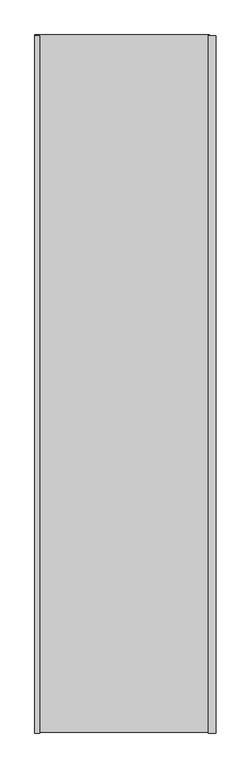
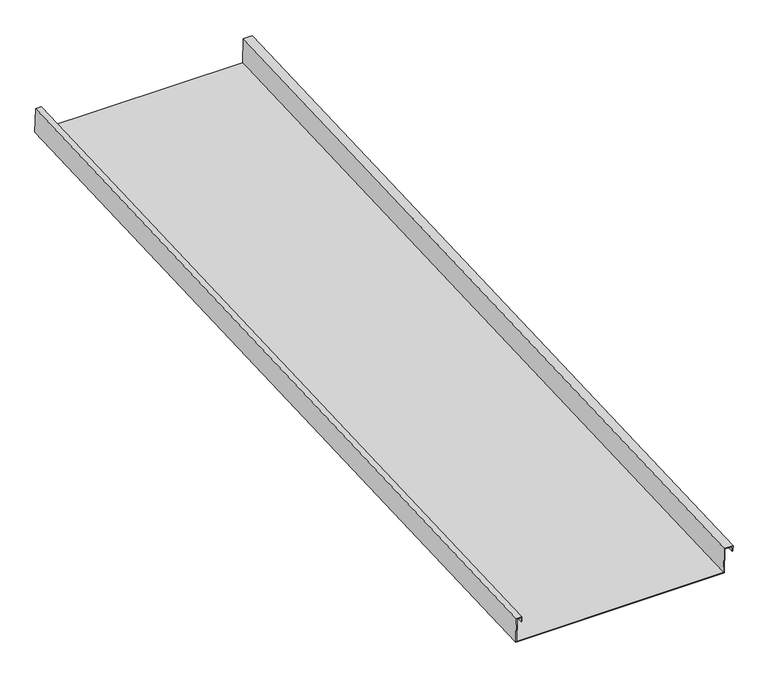
"""IFC4 building model written with IfcOpenShell, lengths in millimetres: proxy geometry, Generic Models 2:Generic Models 2:310765:Generic Models 2:310765 : Generic Models 2:Generic Models 2:310765:62 : Generic Models 2:Generic Models 2:310765:Generic Models 2:310765 : Generic Models 2:Generic Models 2:310765:300385."""

import ifcopenshell
import ifcopenshell.guid

model = None  # the IFC model being written
_history = None  # IfcOwnerHistory: only IFC2X3 demands one
_inside = {}  # id of a spatial element -> (the spatial element, [elements in it])
_under = {}  # id of a project, library or spatial element -> (it, [spatial elements below it])
_declared = {}  # id of a project -> (the project, [libraries it declares])
_typed = {}  # id of a type object -> (the type object, [elements of that type])
_made_of = {}  # id of a material, layer set ... -> (it, [elements and type objects made of it])


def new_model(schema):
    """Start an empty IFC model of exactly this schema.

    Asked for "IFC4X3", IfcOpenShell would pick the latest addendum, in which some entities
    have other attributes; the version numbers below select the first issue.
    IFC2X3 requires an IfcOwnerHistory on every rooted entity: one is made here for all.
    """
    global model, _history
    if schema == "IFC4X3":
        model = ifcopenshell.file(schema_version=(4, 3, 0, 0))
    else:
        model = ifcopenshell.file(schema=schema)
    _inside.clear()
    _under.clear()
    _declared.clear()
    _typed.clear()
    _made_of.clear()
    _history = None
    if model.schema == "IFC2X3":
        org = make("IfcOrganization", Name="unknown")
        user = make(
            "IfcPersonAndOrganization",
            ThePerson=make("IfcPerson", FamilyName="unknown"),
            TheOrganization=org,
        )
        app = make(
            "IfcApplication",
            ApplicationDeveloper=org,
            Version="unknown",
            ApplicationFullName="unknown",
            ApplicationIdentifier="unknown",
        )
        _history = make(
            "IfcOwnerHistory",
            OwningUser=user,
            OwningApplication=app,
            ChangeAction="ADDED",
            CreationDate=0,
        )
    return model


def make(cls, **values):
    """One entity of the class cls with the attributes given. An attribute that is None is left unset."""
    return model.create_entity(
        cls, **{name: value for name, value in values.items() if value is not None}
    )


def rooted(cls, **values):
    """An entity with a GlobalId (a new one), such as an element, a storey or a relation."""
    return make(cls, GlobalId=ifcopenshell.guid.new(), OwnerHistory=_history, **values)


def si_unit(unit_type, name, prefix=None):
    """IfcSIUnit, for example si_unit("LENGTHUNIT", "METRE", prefix="MILLI")."""
    return make("IfcSIUnit", UnitType=unit_type, Prefix=prefix, Name=name)


def assignment(units):
    """IfcUnitAssignment: the units of a project."""
    return None if units is None else make("IfcUnitAssignment", Units=units)


def point(xyz):
    """IfcCartesianPoint."""
    return None if xyz is None else make("IfcCartesianPoint", Coordinates=xyz)


def direction(xyz):
    """IfcDirection."""
    return None if xyz is None else make("IfcDirection", DirectionRatios=xyz)


def frame(location, z_axis=None, x_axis=None):
    """IfcAxis2Placement3D, a coordinate frame: its origin and axes. An axis left out is left unset."""
    return make(
        "IfcAxis2Placement3D",
        Location=point(location),
        Axis=direction(z_axis),
        RefDirection=direction(x_axis),
    )


def origin():
    """The frame at (0, 0, 0) with its axes left unset."""
    return frame((0.0, 0.0, 0.0))


def place(relative_to, where):
    """IfcLocalPlacement: puts the frame where relative to a parent placement (None: the world)."""
    return make(
        "IfcLocalPlacement", PlacementRelTo=relative_to, RelativePlacement=where
    )


def context(
    kind, dimensions, precision=None, world=None, true_north=None, identifier=None
):
    """IfcGeometricRepresentationContext, for example the 3D "Model" context."""
    return make(
        "IfcGeometricRepresentationContext",
        ContextIdentifier=identifier,
        ContextType=kind,
        CoordinateSpaceDimension=dimensions,
        Precision=precision,
        WorldCoordinateSystem=world,
        TrueNorth=true_north,
    )


def project(units=None, contexts=None):
    """IfcProject with its units and contexts."""
    return rooted(
        "IfcProject",
        Name="project",
        RepresentationContexts=contexts,
        UnitsInContext=assignment(units),
    )


def spatial(cls, under=None, at=None, **own):
    """A site, building, storey or space (cls), placed at a placement, below another one or the project."""
    s = rooted(cls, ObjectPlacement=at, **own)
    if under is not None:
        _under.setdefault(under.id(), (under, []))[1].append(s)
    return s


def polyline(points):
    """IfcPolyline through the points."""
    return make("IfcPolyline", Points=[point(p) for p in points])


def outline(outer, holes=None, kind="AREA"):
    """IfcArbitraryClosedProfileDef: a profile drawn as a closed curve; with holes, ...WithVoids."""
    if holes is None:
        return make("IfcArbitraryClosedProfileDef", ProfileType=kind, OuterCurve=outer)
    return make(
        "IfcArbitraryProfileDefWithVoids",
        ProfileType=kind,
        OuterCurve=outer,
        InnerCurves=holes,
    )


def extrude(swept, where, along, depth):
    """IfcExtrudedAreaSolid: the profile swept, set in the frame where, extruded along a direction by depth."""
    return make(
        "IfcExtrudedAreaSolid",
        SweptArea=swept,
        Position=where,
        ExtrudedDirection=direction(along),
        Depth=depth,
    )


def shape(context_of_items, identifier, shape_type, items):
    """IfcShapeRepresentation: the items that make up one representation, for example the "Body"."""
    return make(
        "IfcShapeRepresentation",
        ContextOfItems=context_of_items,
        RepresentationIdentifier=identifier,
        RepresentationType=shape_type,
        Items=items,
    )


def source(mapping_origin, context_of_items, identifier, shape_type, items):
    """IfcRepresentationMap: a shape defined once, which mapped items show again and again."""
    return make(
        "IfcRepresentationMap",
        MappingOrigin=mapping_origin,
        MappedRepresentation=shape(context_of_items, identifier, shape_type, items),
    )


def transform(
    local_origin,
    x_axis=None,
    y_axis=None,
    z_axis=None,
    scale=None,
    scale2=None,
    scale3=None,
    uniform=True,
):
    """IfcCartesianTransformationOperator3D, or its non-uniform kind. x_axis, y_axis, z_axis: its Axis1, 2, 3."""
    if uniform:
        return make(
            "IfcCartesianTransformationOperator3D",
            Axis1=direction(x_axis),
            Axis2=direction(y_axis),
            LocalOrigin=point(local_origin),
            Scale=scale,
            Axis3=direction(z_axis),
        )
    return make(
        "IfcCartesianTransformationOperator3DnonUniform",
        Axis1=direction(x_axis),
        Axis2=direction(y_axis),
        LocalOrigin=point(local_origin),
        Scale=scale,
        Axis3=direction(z_axis),
        Scale2=scale2,
        Scale3=scale3,
    )


def mapped(mapping_source, mapping_target):
    """IfcMappedItem: shows the shape of a source again, moved by a transform."""
    return make(
        "IfcMappedItem", MappingSource=mapping_source, MappingTarget=mapping_target
    )


def made_of(thing, what):
    """Note that an element or type object is made of a material, layer set ...; save() writes the relation."""
    if what is not None:
        _made_of.setdefault(what.id(), (what, []))[1].append(thing)
    return thing


def element(
    cls,
    number,
    at=None,
    inside=None,
    cuts=None,
    type_object=None,
    material=None,
    context=None,
    identifier="Body",
    shape_type=None,
    held_by="IfcProductDefinitionShape",
    body=None,
    shapes=None,
    **own,
):
    """One element of the class cls, such as IfcWall. Its Tag is "e" and its number.

    at: its placement. inside: the storey or other place that contains it. cuts: it is an
    opening in that element (IfcRelVoidsElement). A single representation is given by context,
    identifier, shape_type and body (its items); several are given by shapes. held_by: the class
    of the entity that holds the representations. save() writes the other relations.
    """
    e = rooted(cls, Tag="e%d" % number, ObjectPlacement=at, **own)
    if body is not None:
        shapes = [shape(context, identifier, shape_type, body)]
    if shapes is not None:
        e.Representation = make(held_by, Representations=shapes)
    if inside is not None:
        _inside.setdefault(inside.id(), (inside, []))[1].append(e)
    if cuts is not None:
        rooted(
            "IfcRelVoidsElement", RelatingBuildingElement=cuts, RelatedOpeningElement=e
        )
    if type_object is not None:
        _typed.setdefault(type_object.id(), (type_object, []))[1].append(e)
    return made_of(e, material)


def aggregate(whole, parts):
    """IfcRelAggregates: a whole, such as a stair, and the parts it consists of."""
    return rooted("IfcRelAggregates", RelatingObject=whole, RelatedObjects=parts)


def save(model, path):
    """Write the relations noted so far, then the file.

    IfcRelAggregates (storeys below a building ...), IfcRelContainedInSpatialStructure (elements
    in a storey), IfcRelDefinesByType, IfcRelAssociatesMaterial and IfcRelDeclares: one each for
    every whole, place, type object, material and project.
    """
    for whole, parts in _under.values():
        aggregate(whole, parts)
    for where, things in _inside.values():
        rooted(
            "IfcRelContainedInSpatialStructure",
            RelatedElements=things,
            RelatingStructure=where,
        )
    for kind, things in _typed.values():
        rooted("IfcRelDefinesByType", RelatedObjects=things, RelatingType=kind)
    for what, things in _made_of.values():
        rooted("IfcRelAssociatesMaterial", RelatedObjects=things, RelatingMaterial=what)
    for by, libraries in _declared.values():
        rooted("IfcRelDeclares", RelatingContext=by, RelatedDefinitions=libraries)
    model.write(path)


def generic_models_d106d9bd(model_context):
    return source(origin(), model_context, "Body", "SweptSolid", [
        extrude(outline(polyline([(50.8, 0.0), (50.8, 14.2875), (41.275, 14.2875), (41.275, 15.875), (52.3875, 15.875), (52.3875, -1.5875), (1.5874999, -1.5875), (1.5874999, -404.8125), (47.625, -404.8125), (47.625, -396.875), (39.6875, -396.875), (39.6875, -395.2875), (49.2125, -395.2875), (49.2125, -406.4), (0.0, -406.4), (0.0, 0.0), (50.8, 0.0)])), frame((579172.0218144, -580678.4204475, 3889.8483266), z_axis=(0.0, 0.9991330730923567, 0.04163054471206783), x_axis=(0.0, -0.04163054471206783, 0.9991330730923567)), (0.0, 0.0, 1.0), 1623.6955874),
    ])


if __name__ == "__main__":
    model = new_model("IFC4")
    model_context = context("Model", 3, world=origin())
    ifc_project = project(units=[si_unit("LENGTHUNIT", "METRE", prefix="MILLI")], contexts=[model_context])
    site = spatial("IfcSite", under=ifc_project)
    building = spatial("IfcBuilding", under=site)
    placement = place(None, origin())
    generic_models_shape = generic_models_d106d9bd(model_context)
    element("IfcBuildingElementProxy", 1, Name="Generic Models 2:Generic Models 2:310765:Generic Models 2:310765 : Generic Models 2:Generic Models 2:310765:62 : Generic Models 2:Generic Models 2:310765:Generic Models 2:310765 : Generic Models 2:Generic Models 2:310765:300385", ObjectType="Generic Models 2:Generic Models 2:310765:Generic Models 2:310765 : Generic Models 2:Generic Models 2:310765:62 : Generic Models 2:Generic Models 2:310765:Generic Models 2:310765 : Generic Models 2:Generic Models 2:310765:300385", at=placement, inside=building, context=model_context, shape_type="MappedRepresentation", body=[
        mapped(generic_models_shape, transform((0.0, 0.0, 0.0), x_axis=(1.0, 0.0, 0.0), y_axis=(0.0, 1.0, 0.0), z_axis=(0.0, 0.0, 1.0))),
    ])
    save(model, "model.ifc")

# Revit data of these elements
# Type "Generic Models 2:Generic Models 2:310765:Generic Models 2:310765 : Generic Models 2:Generic Models 2:310765:62 : Generic Models 2:Generic Models 2:310765:Generic Models 2:310765 : Generic Models 2:Generic Models 2:310765:300385"
#   NameOverride = "Generic Models 2:Generic Models 2:310765:Generic Models 2:310765 : Generic Models 2:Generic Models 2:310765:300385"
#   ObjectTypeOverride = "Generic Models 2:310765 : Generic Models 2:Generic Models 2:310765"
#   Reference = "Generic Models 2"
#   Tag = "300385"
# Element 1 (IfcBuildingElementProxy, "Generic Models 2:Generic Models 2:310765:Generic Models 2:310765 : Generic Models 2:Generic Models 2:310765:62 : Generic Models 2:Generic Models 2:310765:Generic Models 2:310765 : Generic Models 2:Generic Models 2:310765:300385")
#   Materials on its faces: "STRUCTURAL STANDING SEAM SHEET METAL ROOFING - BATTENLOK - COLOR T.B.D."
# Materials
#   "STRUCTURAL STANDING SEAM SHEET METAL ROOFING - BATTENLOK - COLOR T.B.D.": class "Generic", colour RGB 120 120 120, transparency 0, Cost = 0
